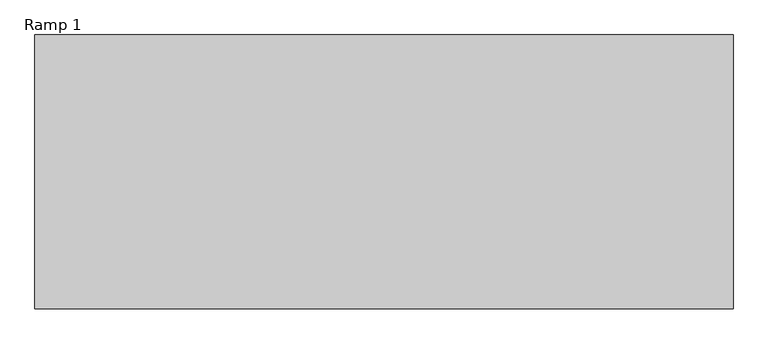
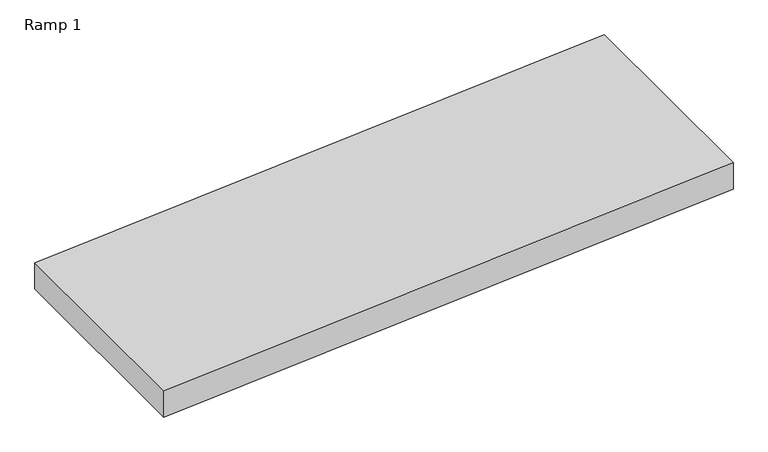
"""IFC4 building model written with IfcOpenShell, lengths in millimetres: ramp geometry, Ramp 1."""

from ifc_helpers import new_model, si_unit, frame, origin, place, context, project, spatial, polyline, outline, extrude, source, transform, mapped, element, save


def ramp_1_ce501800(model_context):
    return source(origin(), model_context, "Body", "SweptSolid", [
        extrude(outline(polyline([(0.0, -7500.2064028), (-225.0, -10560.2064028), (-375.4049465, -10560.2064028), (-150.4049465, -7500.2064028), (0.0, -7500.2064028)])), frame((0.0, -1636.162817, 0.0), z_axis=(0.0, 1.0, 0.0), x_axis=(0.0, 0.0, 1.0)), (0.0, 0.0, 1.0), 1200.0),
    ])


if __name__ == "__main__":
    model = new_model("IFC4")
    model_context = context("Model", 3, world=origin())
    ifc_project = project(units=[si_unit("LENGTHUNIT", "METRE", prefix="MILLI")], contexts=[model_context])
    site = spatial("IfcSite", under=ifc_project)
    building = spatial("IfcBuilding", under=site)
    placement = place(None, origin())
    ramp_1_shape = ramp_1_ce501800(model_context)
    element("IfcRamp", 1, ObjectType="Ramp 1", at=placement, inside=building, context=model_context, shape_type="MappedRepresentation", body=[
        mapped(ramp_1_shape, transform((0.0, 0.0, 0.0), x_axis=(1.0, 0.0, 0.0), y_axis=(0.0, 1.0, 0.0), z_axis=(0.0, 0.0, 1.0))),
    ])
    save(model, "model.ifc")

# Revit data of these elements
# Element 1 (IfcRamp, "Ramp 1")
#   Materials on its faces: "Concrete, Cast In Situ"
# Materials
#   "Concrete, Cast In Situ": class "Concrete", colour RGB 192 192 192, transparency 0, Keynote = "F30/110", Description = "physical material", Cost = 0
